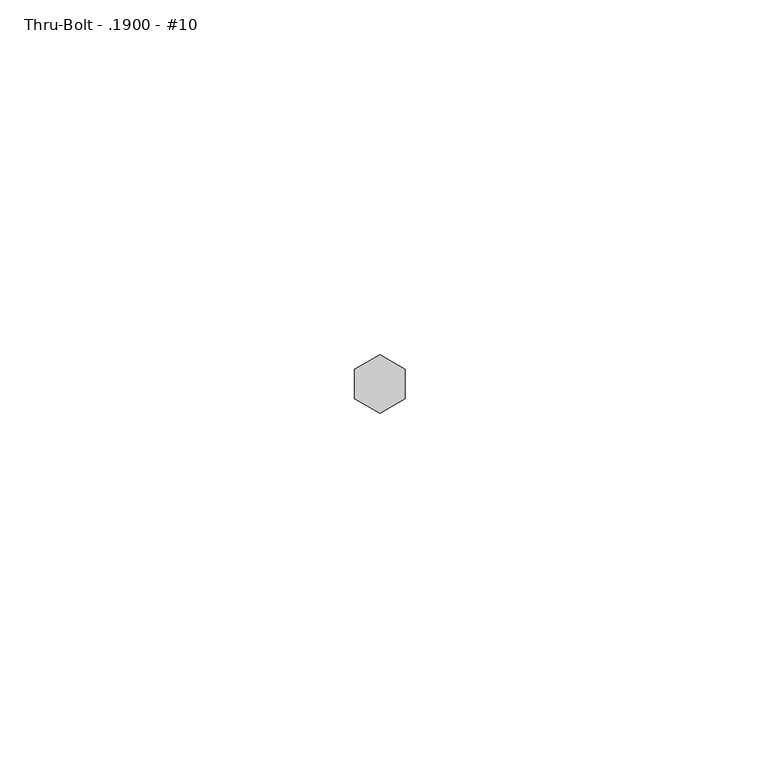
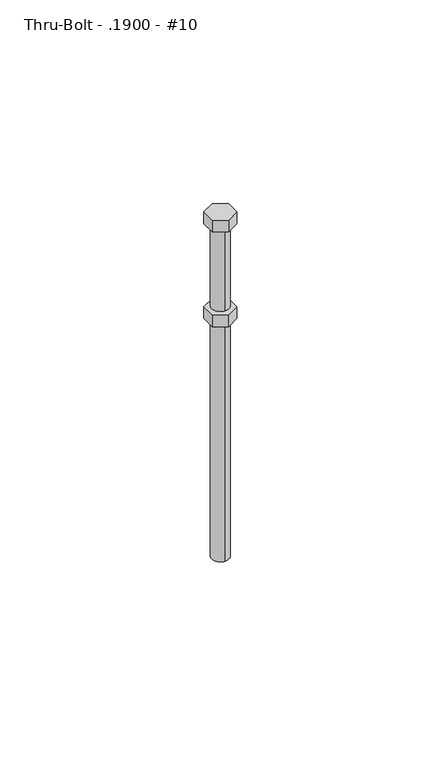
"""IFC4 building model written with IfcOpenShell, lengths in millimetres: fastener geometry, 060523 - W_P_C - Fastenings - Generic : Thru-Bolt - .1900 - #10."""

import ifcopenshell
import ifcopenshell.guid

model = None  # the IFC model being written
_history = None  # IfcOwnerHistory: only IFC2X3 demands one
_inside = {}  # id of a spatial element -> (the spatial element, [elements in it])
_under = {}  # id of a project, library or spatial element -> (it, [spatial elements below it])
_declared = {}  # id of a project -> (the project, [libraries it declares])
_typed = {}  # id of a type object -> (the type object, [elements of that type])
_made_of = {}  # id of a material, layer set ... -> (it, [elements and type objects made of it])


def new_model(schema):
    """Start an empty IFC model of exactly this schema.

    Asked for "IFC4X3", IfcOpenShell would pick the latest addendum, in which some entities
    have other attributes; the version numbers below select the first issue.
    IFC2X3 requires an IfcOwnerHistory on every rooted entity: one is made here for all.
    """
    global model, _history
    if schema == "IFC4X3":
        model = ifcopenshell.file(schema_version=(4, 3, 0, 0))
    else:
        model = ifcopenshell.file(schema=schema)
    _inside.clear()
    _under.clear()
    _declared.clear()
    _typed.clear()
    _made_of.clear()
    _history = None
    if model.schema == "IFC2X3":
        org = make("IfcOrganization", Name="unknown")
        user = make(
            "IfcPersonAndOrganization",
            ThePerson=make("IfcPerson", FamilyName="unknown"),
            TheOrganization=org,
        )
        app = make(
            "IfcApplication",
            ApplicationDeveloper=org,
            Version="unknown",
            ApplicationFullName="unknown",
            ApplicationIdentifier="unknown",
        )
        _history = make(
            "IfcOwnerHistory",
            OwningUser=user,
            OwningApplication=app,
            ChangeAction="ADDED",
            CreationDate=0,
        )
    return model


def make(cls, **values):
    """One entity of the class cls with the attributes given. An attribute that is None is left unset."""
    return model.create_entity(
        cls, **{name: value for name, value in values.items() if value is not None}
    )


def rooted(cls, **values):
    """An entity with a GlobalId (a new one), such as an element, a storey or a relation."""
    return make(cls, GlobalId=ifcopenshell.guid.new(), OwnerHistory=_history, **values)


def si_unit(unit_type, name, prefix=None):
    """IfcSIUnit, for example si_unit("LENGTHUNIT", "METRE", prefix="MILLI")."""
    return make("IfcSIUnit", UnitType=unit_type, Prefix=prefix, Name=name)


def assignment(units):
    """IfcUnitAssignment: the units of a project."""
    return None if units is None else make("IfcUnitAssignment", Units=units)


def point(xyz):
    """IfcCartesianPoint."""
    return None if xyz is None else make("IfcCartesianPoint", Coordinates=xyz)


def direction(xyz):
    """IfcDirection."""
    return None if xyz is None else make("IfcDirection", DirectionRatios=xyz)


def frame(location, z_axis=None, x_axis=None):
    """IfcAxis2Placement3D, a coordinate frame: its origin and axes. An axis left out is left unset."""
    return make(
        "IfcAxis2Placement3D",
        Location=point(location),
        Axis=direction(z_axis),
        RefDirection=direction(x_axis),
    )


def frame_2d(location, x_axis=None):
    """IfcAxis2Placement2D, a coordinate frame in the plane: its origin and x axis."""
    return make(
        "IfcAxis2Placement2D", Location=point(location), RefDirection=direction(x_axis)
    )


def origin():
    """The frame at (0, 0, 0) with its axes left unset."""
    return frame((0.0, 0.0, 0.0))


def origin_with_axes():
    """The frame at (0, 0, 0) with the z axis (0, 0, 1) and the x axis (1, 0, 0) written out."""
    return frame((0.0, 0.0, 0.0), z_axis=(0.0, 0.0, 1.0), x_axis=(1.0, 0.0, 0.0))


def origin_2d():
    """The frame at (0, 0) in the plane with its x axis left unset."""
    return frame_2d((0.0, 0.0))


def place(relative_to, where):
    """IfcLocalPlacement: puts the frame where relative to a parent placement (None: the world)."""
    return make(
        "IfcLocalPlacement", PlacementRelTo=relative_to, RelativePlacement=where
    )


def context(
    kind, dimensions, precision=None, world=None, true_north=None, identifier=None
):
    """IfcGeometricRepresentationContext, for example the 3D "Model" context."""
    return make(
        "IfcGeometricRepresentationContext",
        ContextIdentifier=identifier,
        ContextType=kind,
        CoordinateSpaceDimension=dimensions,
        Precision=precision,
        WorldCoordinateSystem=world,
        TrueNorth=true_north,
    )


def project(units=None, contexts=None):
    """IfcProject with its units and contexts."""
    return rooted(
        "IfcProject",
        Name="project",
        RepresentationContexts=contexts,
        UnitsInContext=assignment(units),
    )


def spatial(cls, under=None, at=None, **own):
    """A site, building, storey or space (cls), placed at a placement, below another one or the project."""
    s = rooted(cls, ObjectPlacement=at, **own)
    if under is not None:
        _under.setdefault(under.id(), (under, []))[1].append(s)
    return s


def polyline(points):
    """IfcPolyline through the points."""
    return make("IfcPolyline", Points=[point(p) for p in points])


def circle_curve(where, radius):
    """IfcCircle in the frame where."""
    return make("IfcCircle", Position=where, Radius=radius)


def trimmed(basis, trim1, trim2, sense, master):
    """IfcTrimmedCurve: the piece of a basis curve between two trims."""
    return make(
        "IfcTrimmedCurve",
        BasisCurve=basis,
        Trim1=trim1,
        Trim2=trim2,
        SenseAgreement=sense,
        MasterRepresentation=master,
    )


def segment(curve, same_sense, transition):
    """IfcCompositeCurveSegment."""
    return make(
        "IfcCompositeCurveSegment",
        Transition=transition,
        SameSense=same_sense,
        ParentCurve=curve,
    )


def composite_curve(segments, self_intersect=None):
    """IfcCompositeCurve: segments joined end to end."""
    return make("IfcCompositeCurve", Segments=segments, SelfIntersect=self_intersect)


def outline(outer, holes=None, kind="AREA"):
    """IfcArbitraryClosedProfileDef: a profile drawn as a closed curve; with holes, ...WithVoids."""
    if holes is None:
        return make("IfcArbitraryClosedProfileDef", ProfileType=kind, OuterCurve=outer)
    return make(
        "IfcArbitraryProfileDefWithVoids",
        ProfileType=kind,
        OuterCurve=outer,
        InnerCurves=holes,
    )


def extrude(swept, where, along, depth):
    """IfcExtrudedAreaSolid: the profile swept, set in the frame where, extruded along a direction by depth."""
    return make(
        "IfcExtrudedAreaSolid",
        SweptArea=swept,
        Position=where,
        ExtrudedDirection=direction(along),
        Depth=depth,
    )


def shape(context_of_items, identifier, shape_type, items):
    """IfcShapeRepresentation: the items that make up one representation, for example the "Body"."""
    return make(
        "IfcShapeRepresentation",
        ContextOfItems=context_of_items,
        RepresentationIdentifier=identifier,
        RepresentationType=shape_type,
        Items=items,
    )


def source(mapping_origin, context_of_items, identifier, shape_type, items):
    """IfcRepresentationMap: a shape defined once, which mapped items show again and again."""
    return make(
        "IfcRepresentationMap",
        MappingOrigin=mapping_origin,
        MappedRepresentation=shape(context_of_items, identifier, shape_type, items),
    )


def transform(
    local_origin,
    x_axis=None,
    y_axis=None,
    z_axis=None,
    scale=None,
    scale2=None,
    scale3=None,
    uniform=True,
):
    """IfcCartesianTransformationOperator3D, or its non-uniform kind. x_axis, y_axis, z_axis: its Axis1, 2, 3."""
    if uniform:
        return make(
            "IfcCartesianTransformationOperator3D",
            Axis1=direction(x_axis),
            Axis2=direction(y_axis),
            LocalOrigin=point(local_origin),
            Scale=scale,
            Axis3=direction(z_axis),
        )
    return make(
        "IfcCartesianTransformationOperator3DnonUniform",
        Axis1=direction(x_axis),
        Axis2=direction(y_axis),
        LocalOrigin=point(local_origin),
        Scale=scale,
        Axis3=direction(z_axis),
        Scale2=scale2,
        Scale3=scale3,
    )


def mapped(mapping_source, mapping_target):
    """IfcMappedItem: shows the shape of a source again, moved by a transform."""
    return make(
        "IfcMappedItem", MappingSource=mapping_source, MappingTarget=mapping_target
    )


def made_of(thing, what):
    """Note that an element or type object is made of a material, layer set ...; save() writes the relation."""
    if what is not None:
        _made_of.setdefault(what.id(), (what, []))[1].append(thing)
    return thing


def element(
    cls,
    number,
    at=None,
    inside=None,
    cuts=None,
    type_object=None,
    material=None,
    context=None,
    identifier="Body",
    shape_type=None,
    held_by="IfcProductDefinitionShape",
    body=None,
    shapes=None,
    **own,
):
    """One element of the class cls, such as IfcWall. Its Tag is "e" and its number.

    at: its placement. inside: the storey or other place that contains it. cuts: it is an
    opening in that element (IfcRelVoidsElement). A single representation is given by context,
    identifier, shape_type and body (its items); several are given by shapes. held_by: the class
    of the entity that holds the representations. save() writes the other relations.
    """
    e = rooted(cls, Tag="e%d" % number, ObjectPlacement=at, **own)
    if body is not None:
        shapes = [shape(context, identifier, shape_type, body)]
    if shapes is not None:
        e.Representation = make(held_by, Representations=shapes)
    if inside is not None:
        _inside.setdefault(inside.id(), (inside, []))[1].append(e)
    if cuts is not None:
        rooted(
            "IfcRelVoidsElement", RelatingBuildingElement=cuts, RelatedOpeningElement=e
        )
    if type_object is not None:
        _typed.setdefault(type_object.id(), (type_object, []))[1].append(e)
    return made_of(e, material)


def aggregate(whole, parts):
    """IfcRelAggregates: a whole, such as a stair, and the parts it consists of."""
    return rooted("IfcRelAggregates", RelatingObject=whole, RelatedObjects=parts)


def save(model, path):
    """Write the relations noted so far, then the file.

    IfcRelAggregates (storeys below a building ...), IfcRelContainedInSpatialStructure (elements
    in a storey), IfcRelDefinesByType, IfcRelAssociatesMaterial and IfcRelDeclares: one each for
    every whole, place, type object, material and project.
    """
    for whole, parts in _under.values():
        aggregate(whole, parts)
    for where, things in _inside.values():
        rooted(
            "IfcRelContainedInSpatialStructure",
            RelatedElements=things,
            RelatingStructure=where,
        )
    for kind, things in _typed.values():
        rooted("IfcRelDefinesByType", RelatedObjects=things, RelatingType=kind)
    for what, things in _made_of.values():
        rooted("IfcRelAssociatesMaterial", RelatedObjects=things, RelatingMaterial=what)
    for by, libraries in _declared.values():
        rooted("IfcRelDeclares", RelatingContext=by, RelatedDefinitions=libraries)
    model.write(path)


def thru_bolt_1900_10_47653ec8(model_context):
    return source(origin(), model_context, "Body", "SweptSolid", [
        extrude(outline(polyline([(-3.571875, -2.062223), (-3.571875, 2.062223), (0.0, 4.124446), (3.571875, 2.062223), (3.571875, -2.062223), (0.0, -4.124446), (-3.571875, -2.062223)])), frame((0.0, 0.0, -28.971875), z_axis=(0.0, 0.0, 1.0), x_axis=(1.0, 0.0, 0.0)), (0.0, 0.0, 1.0), 3.571875),
        extrude(outline(polyline([(-3.571875, 2.062223), (0.0, 4.124446), (3.571875, 2.062223), (3.571875, -2.062223), (0.0, -4.124446), (-3.571875, -2.062223), (-3.571875, 2.062223)])), origin_with_axes(), (0.0, 0.0, 1.0), 3.571875),
        extrude(outline(composite_curve([segment(trimmed(circle_curve(origin_2d(), 2.5300781), [point((0.0, -2.5300781))], [point((0.0, 2.5300781))], False, "CARTESIAN"), True, "CONTINUOUS"), segment(trimmed(circle_curve(origin_2d(), 2.5300781), [point((0.0, 2.5300781))], [point((0.0, -2.5300781))], False, "CARTESIAN"), True, "CONTINUOUS")], self_intersect=False)), frame((0.0, 0.0, -101.6), z_axis=(0.0, 0.0, 1.0), x_axis=(1.0, 0.0, 0.0)), (0.0, 0.0, 1.0), 101.6),
    ])


if __name__ == "__main__":
    model = new_model("IFC4")
    model_context = context("Model", 3, world=origin())
    ifc_project = project(units=[si_unit("LENGTHUNIT", "METRE", prefix="MILLI")], contexts=[model_context])
    site = spatial("IfcSite", under=ifc_project)
    building = spatial("IfcBuilding", under=site)
    placement = place(None, origin())
    thru_bolt_1900_10_shape = thru_bolt_1900_10_47653ec8(model_context)
    element("IfcFastener", 1, ObjectType="060523 - W_P_C - Fastenings - Generic : Thru-Bolt - .1900 - #10", at=placement, inside=building, context=model_context, shape_type="MappedRepresentation", body=[
        mapped(thru_bolt_1900_10_shape, transform((0.0, 0.0, 0.0), x_axis=(1.0, 0.0, 0.0), y_axis=(0.0, 1.0, 0.0), z_axis=(0.0, 0.0, 1.0))),
    ])
    save(model, "model.ifc")

# Revit data of these elements
# Type "060523 - W_P_C - Fastenings - Generic : Thru-Bolt - .1900 - #10"
#   Washer_Thickness = 0' - 0 3/64"
#   Washer Radius = 0' - 0.24023"
#   Washer Offset - Head = 0' - 0"
#   Washer Offset = 0' - 0"
#   Thickness_of_Substrate [instance default] = 0' - 1"
#   Side = 0' - 0.1626"
#   Radius = 0' - 0.09961"
#   Length [instance default] = 0' - 4"
#   Head Size = 0' - 0 9/32"
#   Head Radius = 0' - 0 9/64"
#   Head Height = 0' - 0 9/64"
#   Double Diameter = 0' - 0 51/128"
#   Diameter = 0' - 0 51/256"
#   Default Elevation = 4' - 0"
#   Washer_Nut_Visibility = no
#   Washer_Head_Visibility = no
#   Round_Head_Visibility = no
#   Point Visibility = no
#   Nut_Visibility = yes
#   Hex_Head_Visiblilty = yes
#   Washer Material = none
#   Bolt Material (Size) = AT SILL - FASTENER AT 24" O.C.
# Element 1 (IfcFastener, "060523 - W_P_C - Fastenings - Generic : Thru-Bolt - .1900 - #10")
#   Materials on its faces: "AT SILL - FASTENER AT 24\" O.C."
# Materials
#   "AT SILL - FASTENER AT 24\" O.C.": class "Generic", colour RGB 120 120 120, transparency 0, Cost = 0
